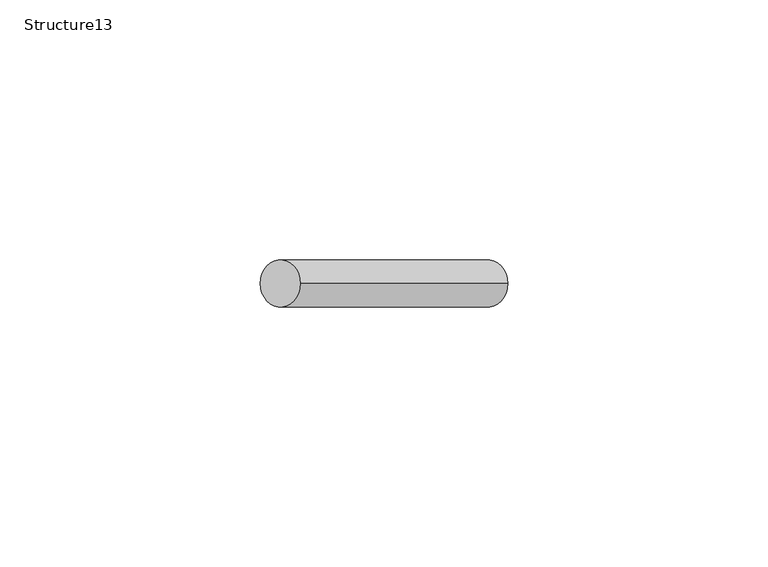
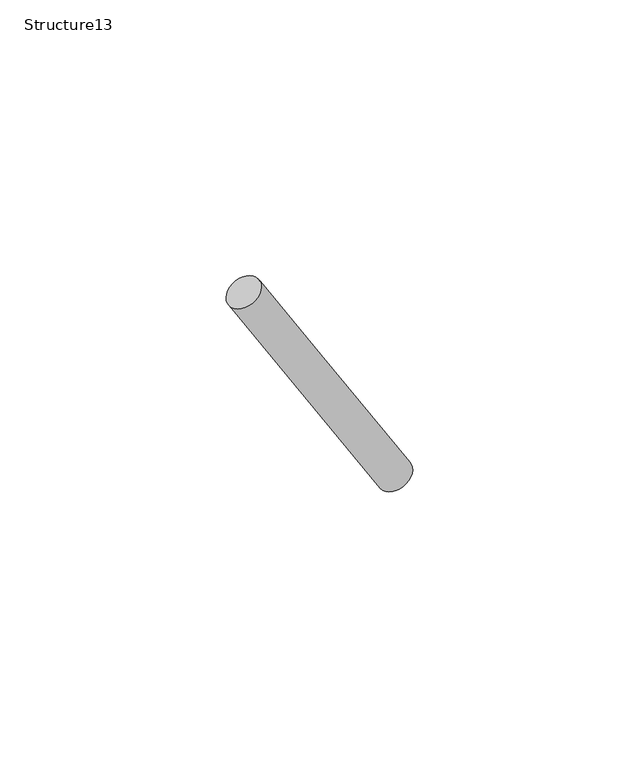
"""IFC4 building model written with IfcOpenShell, lengths in millimetres: proxy geometry, Structure13 : Structure668217134."""

import ifcopenshell
import ifcopenshell.guid

model = None  # the IFC model being written
_history = None  # IfcOwnerHistory: only IFC2X3 demands one
_inside = {}  # id of a spatial element -> (the spatial element, [elements in it])
_under = {}  # id of a project, library or spatial element -> (it, [spatial elements below it])
_declared = {}  # id of a project -> (the project, [libraries it declares])
_typed = {}  # id of a type object -> (the type object, [elements of that type])
_made_of = {}  # id of a material, layer set ... -> (it, [elements and type objects made of it])


def new_model(schema):
    """Start an empty IFC model of exactly this schema.

    Asked for "IFC4X3", IfcOpenShell would pick the latest addendum, in which some entities
    have other attributes; the version numbers below select the first issue.
    IFC2X3 requires an IfcOwnerHistory on every rooted entity: one is made here for all.
    """
    global model, _history
    if schema == "IFC4X3":
        model = ifcopenshell.file(schema_version=(4, 3, 0, 0))
    else:
        model = ifcopenshell.file(schema=schema)
    _inside.clear()
    _under.clear()
    _declared.clear()
    _typed.clear()
    _made_of.clear()
    _history = None
    if model.schema == "IFC2X3":
        org = make("IfcOrganization", Name="unknown")
        user = make(
            "IfcPersonAndOrganization",
            ThePerson=make("IfcPerson", FamilyName="unknown"),
            TheOrganization=org,
        )
        app = make(
            "IfcApplication",
            ApplicationDeveloper=org,
            Version="unknown",
            ApplicationFullName="unknown",
            ApplicationIdentifier="unknown",
        )
        _history = make(
            "IfcOwnerHistory",
            OwningUser=user,
            OwningApplication=app,
            ChangeAction="ADDED",
            CreationDate=0,
        )
    return model


def make(cls, **values):
    """One entity of the class cls with the attributes given. An attribute that is None is left unset."""
    return model.create_entity(
        cls, **{name: value for name, value in values.items() if value is not None}
    )


def rooted(cls, **values):
    """An entity with a GlobalId (a new one), such as an element, a storey or a relation."""
    return make(cls, GlobalId=ifcopenshell.guid.new(), OwnerHistory=_history, **values)


def si_unit(unit_type, name, prefix=None):
    """IfcSIUnit, for example si_unit("LENGTHUNIT", "METRE", prefix="MILLI")."""
    return make("IfcSIUnit", UnitType=unit_type, Prefix=prefix, Name=name)


def assignment(units):
    """IfcUnitAssignment: the units of a project."""
    return None if units is None else make("IfcUnitAssignment", Units=units)


def point(xyz):
    """IfcCartesianPoint."""
    return None if xyz is None else make("IfcCartesianPoint", Coordinates=xyz)


def direction(xyz):
    """IfcDirection."""
    return None if xyz is None else make("IfcDirection", DirectionRatios=xyz)


def frame(location, z_axis=None, x_axis=None):
    """IfcAxis2Placement3D, a coordinate frame: its origin and axes. An axis left out is left unset."""
    return make(
        "IfcAxis2Placement3D",
        Location=point(location),
        Axis=direction(z_axis),
        RefDirection=direction(x_axis),
    )


def frame_2d(location, x_axis=None):
    """IfcAxis2Placement2D, a coordinate frame in the plane: its origin and x axis."""
    return make(
        "IfcAxis2Placement2D", Location=point(location), RefDirection=direction(x_axis)
    )


def origin():
    """The frame at (0, 0, 0) with its axes left unset."""
    return frame((0.0, 0.0, 0.0))


def place(relative_to, where):
    """IfcLocalPlacement: puts the frame where relative to a parent placement (None: the world)."""
    return make(
        "IfcLocalPlacement", PlacementRelTo=relative_to, RelativePlacement=where
    )


def context(
    kind, dimensions, precision=None, world=None, true_north=None, identifier=None
):
    """IfcGeometricRepresentationContext, for example the 3D "Model" context."""
    return make(
        "IfcGeometricRepresentationContext",
        ContextIdentifier=identifier,
        ContextType=kind,
        CoordinateSpaceDimension=dimensions,
        Precision=precision,
        WorldCoordinateSystem=world,
        TrueNorth=true_north,
    )


def project(units=None, contexts=None):
    """IfcProject with its units and contexts."""
    return rooted(
        "IfcProject",
        Name="project",
        RepresentationContexts=contexts,
        UnitsInContext=assignment(units),
    )


def spatial(cls, under=None, at=None, **own):
    """A site, building, storey or space (cls), placed at a placement, below another one or the project."""
    s = rooted(cls, ObjectPlacement=at, **own)
    if under is not None:
        _under.setdefault(under.id(), (under, []))[1].append(s)
    return s


def circle_curve(where, radius):
    """IfcCircle in the frame where."""
    return make("IfcCircle", Position=where, Radius=radius)


def trimmed(basis, trim1, trim2, sense, master):
    """IfcTrimmedCurve: the piece of a basis curve between two trims."""
    return make(
        "IfcTrimmedCurve",
        BasisCurve=basis,
        Trim1=trim1,
        Trim2=trim2,
        SenseAgreement=sense,
        MasterRepresentation=master,
    )


def segment(curve, same_sense, transition):
    """IfcCompositeCurveSegment."""
    return make(
        "IfcCompositeCurveSegment",
        Transition=transition,
        SameSense=same_sense,
        ParentCurve=curve,
    )


def composite_curve(segments, self_intersect=None):
    """IfcCompositeCurve: segments joined end to end."""
    return make("IfcCompositeCurve", Segments=segments, SelfIntersect=self_intersect)


def outline(outer, holes=None, kind="AREA"):
    """IfcArbitraryClosedProfileDef: a profile drawn as a closed curve; with holes, ...WithVoids."""
    if holes is None:
        return make("IfcArbitraryClosedProfileDef", ProfileType=kind, OuterCurve=outer)
    return make(
        "IfcArbitraryProfileDefWithVoids",
        ProfileType=kind,
        OuterCurve=outer,
        InnerCurves=holes,
    )


def extrude(swept, where, along, depth):
    """IfcExtrudedAreaSolid: the profile swept, set in the frame where, extruded along a direction by depth."""
    return make(
        "IfcExtrudedAreaSolid",
        SweptArea=swept,
        Position=where,
        ExtrudedDirection=direction(along),
        Depth=depth,
    )


def shape(context_of_items, identifier, shape_type, items):
    """IfcShapeRepresentation: the items that make up one representation, for example the "Body"."""
    return make(
        "IfcShapeRepresentation",
        ContextOfItems=context_of_items,
        RepresentationIdentifier=identifier,
        RepresentationType=shape_type,
        Items=items,
    )


def source(mapping_origin, context_of_items, identifier, shape_type, items):
    """IfcRepresentationMap: a shape defined once, which mapped items show again and again."""
    return make(
        "IfcRepresentationMap",
        MappingOrigin=mapping_origin,
        MappedRepresentation=shape(context_of_items, identifier, shape_type, items),
    )


def transform(
    local_origin,
    x_axis=None,
    y_axis=None,
    z_axis=None,
    scale=None,
    scale2=None,
    scale3=None,
    uniform=True,
):
    """IfcCartesianTransformationOperator3D, or its non-uniform kind. x_axis, y_axis, z_axis: its Axis1, 2, 3."""
    if uniform:
        return make(
            "IfcCartesianTransformationOperator3D",
            Axis1=direction(x_axis),
            Axis2=direction(y_axis),
            LocalOrigin=point(local_origin),
            Scale=scale,
            Axis3=direction(z_axis),
        )
    return make(
        "IfcCartesianTransformationOperator3DnonUniform",
        Axis1=direction(x_axis),
        Axis2=direction(y_axis),
        LocalOrigin=point(local_origin),
        Scale=scale,
        Axis3=direction(z_axis),
        Scale2=scale2,
        Scale3=scale3,
    )


def mapped(mapping_source, mapping_target):
    """IfcMappedItem: shows the shape of a source again, moved by a transform."""
    return make(
        "IfcMappedItem", MappingSource=mapping_source, MappingTarget=mapping_target
    )


def made_of(thing, what):
    """Note that an element or type object is made of a material, layer set ...; save() writes the relation."""
    if what is not None:
        _made_of.setdefault(what.id(), (what, []))[1].append(thing)
    return thing


def element(
    cls,
    number,
    at=None,
    inside=None,
    cuts=None,
    type_object=None,
    material=None,
    context=None,
    identifier="Body",
    shape_type=None,
    held_by="IfcProductDefinitionShape",
    body=None,
    shapes=None,
    **own,
):
    """One element of the class cls, such as IfcWall. Its Tag is "e" and its number.

    at: its placement. inside: the storey or other place that contains it. cuts: it is an
    opening in that element (IfcRelVoidsElement). A single representation is given by context,
    identifier, shape_type and body (its items); several are given by shapes. held_by: the class
    of the entity that holds the representations. save() writes the other relations.
    """
    e = rooted(cls, Tag="e%d" % number, ObjectPlacement=at, **own)
    if body is not None:
        shapes = [shape(context, identifier, shape_type, body)]
    if shapes is not None:
        e.Representation = make(held_by, Representations=shapes)
    if inside is not None:
        _inside.setdefault(inside.id(), (inside, []))[1].append(e)
    if cuts is not None:
        rooted(
            "IfcRelVoidsElement", RelatingBuildingElement=cuts, RelatedOpeningElement=e
        )
    if type_object is not None:
        _typed.setdefault(type_object.id(), (type_object, []))[1].append(e)
    return made_of(e, material)


def aggregate(whole, parts):
    """IfcRelAggregates: a whole, such as a stair, and the parts it consists of."""
    return rooted("IfcRelAggregates", RelatingObject=whole, RelatedObjects=parts)


def save(model, path):
    """Write the relations noted so far, then the file.

    IfcRelAggregates (storeys below a building ...), IfcRelContainedInSpatialStructure (elements
    in a storey), IfcRelDefinesByType, IfcRelAssociatesMaterial and IfcRelDeclares: one each for
    every whole, place, type object, material and project.
    """
    for whole, parts in _under.values():
        aggregate(whole, parts)
    for where, things in _inside.values():
        rooted(
            "IfcRelContainedInSpatialStructure",
            RelatedElements=things,
            RelatingStructure=where,
        )
    for kind, things in _typed.values():
        rooted("IfcRelDefinesByType", RelatedObjects=things, RelatingType=kind)
    for what, things in _made_of.values():
        rooted("IfcRelAssociatesMaterial", RelatedObjects=things, RelatingMaterial=what)
    for by, libraries in _declared.values():
        rooted("IfcRelDeclares", RelatingContext=by, RelatedDefinitions=libraries)
    model.write(path)


def structure13_aec6eda5(model_context):
    return source(origin(), model_context, "Body", "SweptSolid", [
        extrude(outline(composite_curve([segment(trimmed(circle_curve(frame_2d((0.0, -4.5217365)), 4.5217366), [point((0.0, -9.0434732))], [point((0.0, 0.0))], False, "CARTESIAN"), True, "CONTINUOUS"), segment(trimmed(circle_curve(frame_2d((0.0, -4.5217365)), 4.5217366), [point((0.0, 0.0))], [point((0.0, -9.0434732))], False, "CARTESIAN"), True, "CONTINUOUS")], self_intersect=False)), frame((5198.320189, 1851.7391069, 38035.9872174), z_axis=(-0.523016219738758, 0.0, 0.8523227287185172), x_axis=(0.0, -1.0, 0.0)), (0.0, 0.0, 1.0), 76.2),
    ])


if __name__ == "__main__":
    model = new_model("IFC4")
    model_context = context("Model", 3, world=origin())
    ifc_project = project(units=[si_unit("LENGTHUNIT", "METRE", prefix="MILLI")], contexts=[model_context])
    site = spatial("IfcSite", under=ifc_project)
    building = spatial("IfcBuilding", under=site)
    placement = place(None, origin())
    structure13_shape = structure13_aec6eda5(model_context)
    element("IfcBuildingElementProxy", 1, Name="Structure13 : Structure668217134", ObjectType="Structure13 : Structure668217134", at=placement, inside=building, context=model_context, shape_type="MappedRepresentation", body=[
        mapped(structure13_shape, transform((0.0, 0.0, 0.0), x_axis=(1.0, 0.0, 0.0), y_axis=(0.0, 1.0, 0.0), z_axis=(0.0, 0.0, 1.0))),
    ])
    save(model, "model.ifc")

# Revit data of these elements
# Type "Structure13 : Structure668217134"
#   NameOverride = "Structure668217134"
# Element 1 (IfcBuildingElementProxy, "Structure13 : Structure668217134")
#   Materials on its faces: "1.5\" DIA. STAINLESS STEEL RAILING"
# Materials
#   "1.5\" DIA. STAINLESS STEEL RAILING": class "Unassigned", colour RGB 128 128 128, transparency 0, Cost = 0
